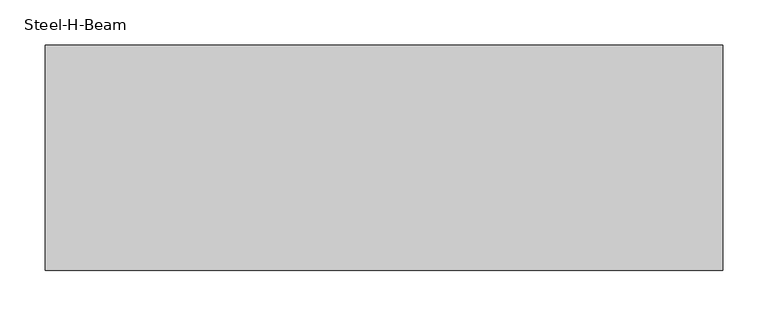
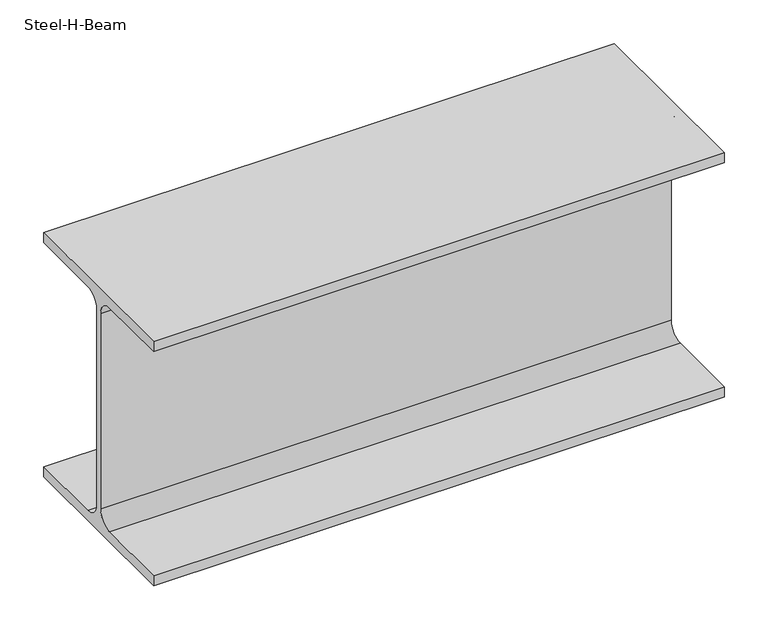
"""IFC4 building model written with IfcOpenShell, lengths in millimetres: beam geometry, Steel-H-Beam : BM121_H-340×250x9x14."""

from ifc_helpers import new_model, si_unit, point, frame, frame_2d, origin, place, context, project, spatial, polyline, circle_curve, trimmed, segment, composite_curve, outline, extrude, source, transform, mapped, element, save


def steel_h_beam_e1c1fa7a(model_context):
    return source(origin(), model_context, "Body", "SweptSolid", [
        extrude(outline(composite_curve([segment(polyline([(125.0, -156.0), (125.0, -170.0), (-125.0, -170.0), (-125.0, -156.0), (-24.5, -156.0)]), True, "CONTINUOUS"), segment(trimmed(circle_curve(frame_2d((-24.5, -136.0)), 20.0), [point((-24.5, -156.0))], [point((-4.5, -136.0))], True, "CARTESIAN"), True, "CONTINUOUS"), segment(polyline([(-4.5, -136.0), (-4.5, 136.0)]), True, "CONTINUOUS"), segment(trimmed(circle_curve(frame_2d((-24.5, 136.0)), 20.0), [point((-4.5, 136.0))], [point((-24.5, 156.0))], True, "CARTESIAN"), True, "CONTINUOUS"), segment(polyline([(-24.5, 156.0), (-125.0, 156.0), (-125.0, 170.0), (125.0, 170.0), (125.0, 156.0), (24.5, 156.0)]), True, "CONTINUOUS"), segment(trimmed(circle_curve(frame_2d((24.5, 136.0)), 20.0), [point((24.5, 156.0))], [point((4.5, 136.0))], True, "CARTESIAN"), True, "CONTINUOUS"), segment(polyline([(4.5, 136.0), (4.5, -136.0)]), True, "CONTINUOUS"), segment(trimmed(circle_curve(frame_2d((24.5, -136.0)), 20.0), [point((4.5, -136.0))], [point((24.5, -156.0))], True, "CARTESIAN"), True, "CONTINUOUS"), segment(polyline([(24.5, -156.0), (125.0, -156.0)]), True, "CONTINUOUS")], self_intersect=False)), frame((-375.3823519, 0.0, 0.0), z_axis=(1.0, 0.0, 0.0), x_axis=(0.0, 1.0, 0.0)), (0.0, 0.0, 1.0), 750.7647038),
    ])


if __name__ == "__main__":
    model = new_model("IFC4")
    model_context = context("Model", 3, world=origin())
    ifc_project = project(units=[si_unit("LENGTHUNIT", "METRE", prefix="MILLI")], contexts=[model_context])
    site = spatial("IfcSite", under=ifc_project)
    building = spatial("IfcBuilding", under=site)
    placement = place(None, origin())
    steel_h_beam_shape = steel_h_beam_e1c1fa7a(model_context)
    element("IfcBeam", 1, ObjectType="Steel-H-Beam : BM121_H-340×250x9x14", at=placement, inside=building, context=model_context, shape_type="MappedRepresentation", body=[
        mapped(steel_h_beam_shape, transform((0.0, 0.0, 0.0), x_axis=(1.0, 0.0, 0.0), y_axis=(0.0, 1.0, 0.0), z_axis=(0.0, 0.0, 1.0))),
    ])
    save(model, "model.ifc")

# Revit data of these elements
# Type "Steel-H-Beam : BM121_H-340×250x9x14"
#   Surface Area = 1.62766 m²/m
#   Section Area = 101.514 cm²
#   Mass per Unit Length = 79.6882 kg/m
#   Length [instance default] = 3000 mm
#   B = 250 mm
#   H = 340 mm
#   r = 20 mm
#   tw = 9 mm
#   tf = 14 mm
#   hec_material4 [instance default] = none
#   hec_material3 [instance default] = none
#   hec_material2 [instance default] = none
#   hec_material1 [instance default] = none
#   Structural Material [instance default] = Steel, 45-345
#   Assembly Code = ""
# Element 1 (IfcBeam, "Steel-H-Beam : BM121_H-340×250x9x14")
#   hec_material3 = F01AC000-00002_Building/Shelter Fire Proofing Work_Intumescent Coating Type_1 hr. rating (UL 1709))
#   hec_material2 = S01AA010-00002_Main Steel Structure Fabrication Work_Shelter/Building_Steel Painting/Coating_for Fireproofed Steel Surface, Surface Preparation & Primer Coat
#   hec_material1 = S03AA028-00001_Main Steel Structure Erection Work_Shelter/Building_Medium Steel
#   Structural Material = S01AA002-00001_Main Steel Structure Fabrication Work_Shelter/Building_Medium Steel - Standard
#   Materials on its faces: "S01AA002-00001_Main Steel Structure Fabrication Work_Shelter/Building_Medium Steel - Standard"
# Materials
#   "Steel, 45-345": class "Metal", colour RGB 189 187 185, transparency 0, Description = "Steel 345 MPa", Cost = 0
#   "S01AA002-00001_Main Steel Structure Fabrication Work_Shelter/Building_Medium Steel - Standard": class "Metal", colour RGB 120 120 120, transparency 0, Comments = "(90KG/M>Weight≥30KG/M)", Description = "Structural steel 50ksi", W00) Work Master Code = "S01AA002-0001", W01) Work Master_Lv1 = "Main Steel Structure Fabrication Work", W02) Work Master_Lv2 = "Shelter/Building", W03) Work Master_Spec.1 = "Medium Steel - Standard (90KG/M>Weight≥30KG/M)", Cost = 0
#   "F01AC000-00002_Building/Shelter Fire Proofing Work_Intumescent Coating Type_1 hr. rating (UL 1709))": class "Metal", colour RGB 255 128 128, transparency 0, Description = "Paint finished steel", W00) Work Master Code = "F01AC000-00002", W01) Work Master_Lv1 = "Building/Shelter Fire Proofing Work", W02) Work Master_Lv2 = "Intumescent Coating Type", W03) Work Master_Spec.1 = "1 hr. rating (UL 1709)", Cost = 0
#   "S01AA010-00002_Main Steel Structure Fabrication Work_Shelter/Building_Steel Painting/Coating_for Fireproofed Steel Surface, Surface Preparation & Primer Coat": class "Metal", colour RGB 120 120 120, transparency 0, Description = "Paint finished steel", W00) Work Master Code = "SS01AA010-00002", W01) Work Master_Lv1 = "Main Steel Structure Fabrication Work", W02) Work Master_Lv2 = "Shelter/Building", W03) Work Master_Spec.1 = "Steel Painting/Coating", W04) Work Master_Spec.2 = "for Fireproofed Steel Surface, Surface Preparation & Primer Coat", Cost = 0
#   "S03AA028-00001_Main Steel Structure Erection Work_Shelter/Building_Medium Steel": class "Metal", colour RGB 120 120 120, transparency 0, Comments = "(90KG/M>Weight≥30KG/M)", Description = "Structural steel 50ksi", W00) Work Master Code = "S03AA028-0001", W01) Work Master_Lv1 = "Main Steel Structure Erection Work", W02) Work Master_Lv2 = "Shelter/Building", W03) Work Master_Spec.1 = "Medium Steel (90KG/M>Weight≥30KG/M)", Cost = 0
